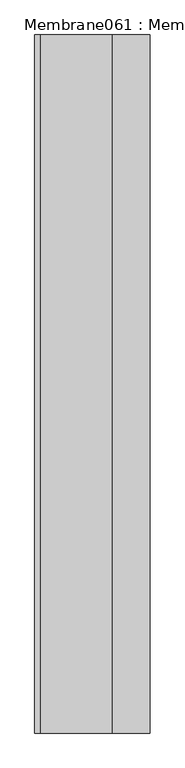
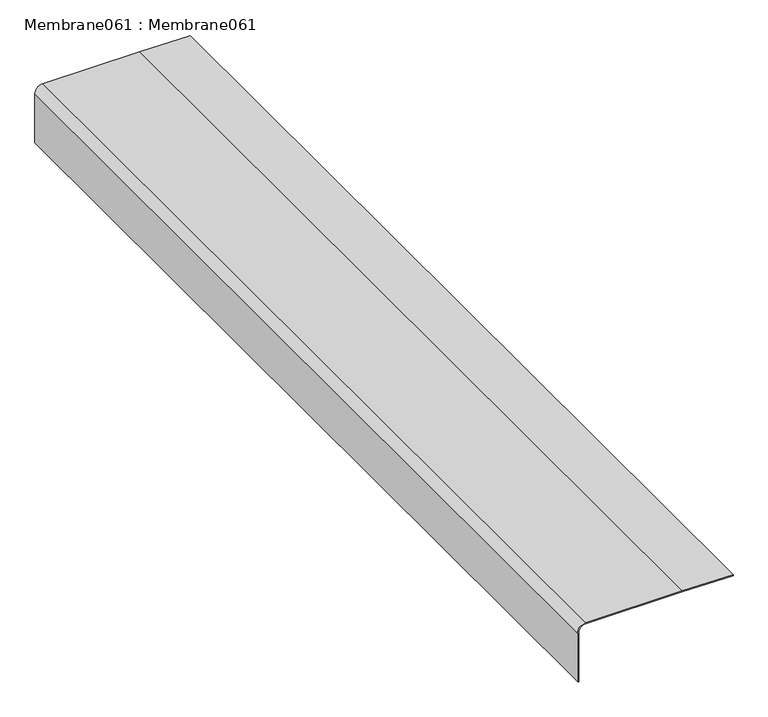
"""IFC4 building model written with IfcOpenShell, lengths in millimetres: proxy geometry, Membrane061 : Membrane061."""

import ifcopenshell
import ifcopenshell.guid

model = None  # the IFC model being written
_history = None  # IfcOwnerHistory: only IFC2X3 demands one
_inside = {}  # id of a spatial element -> (the spatial element, [elements in it])
_under = {}  # id of a project, library or spatial element -> (it, [spatial elements below it])
_declared = {}  # id of a project -> (the project, [libraries it declares])
_typed = {}  # id of a type object -> (the type object, [elements of that type])
_made_of = {}  # id of a material, layer set ... -> (it, [elements and type objects made of it])


def new_model(schema):
    """Start an empty IFC model of exactly this schema.

    Asked for "IFC4X3", IfcOpenShell would pick the latest addendum, in which some entities
    have other attributes; the version numbers below select the first issue.
    IFC2X3 requires an IfcOwnerHistory on every rooted entity: one is made here for all.
    """
    global model, _history
    if schema == "IFC4X3":
        model = ifcopenshell.file(schema_version=(4, 3, 0, 0))
    else:
        model = ifcopenshell.file(schema=schema)
    _inside.clear()
    _under.clear()
    _declared.clear()
    _typed.clear()
    _made_of.clear()
    _history = None
    if model.schema == "IFC2X3":
        org = make("IfcOrganization", Name="unknown")
        user = make(
            "IfcPersonAndOrganization",
            ThePerson=make("IfcPerson", FamilyName="unknown"),
            TheOrganization=org,
        )
        app = make(
            "IfcApplication",
            ApplicationDeveloper=org,
            Version="unknown",
            ApplicationFullName="unknown",
            ApplicationIdentifier="unknown",
        )
        _history = make(
            "IfcOwnerHistory",
            OwningUser=user,
            OwningApplication=app,
            ChangeAction="ADDED",
            CreationDate=0,
        )
    return model


def make(cls, **values):
    """One entity of the class cls with the attributes given. An attribute that is None is left unset."""
    return model.create_entity(
        cls, **{name: value for name, value in values.items() if value is not None}
    )


def rooted(cls, **values):
    """An entity with a GlobalId (a new one), such as an element, a storey or a relation."""
    return make(cls, GlobalId=ifcopenshell.guid.new(), OwnerHistory=_history, **values)


def si_unit(unit_type, name, prefix=None):
    """IfcSIUnit, for example si_unit("LENGTHUNIT", "METRE", prefix="MILLI")."""
    return make("IfcSIUnit", UnitType=unit_type, Prefix=prefix, Name=name)


def assignment(units):
    """IfcUnitAssignment: the units of a project."""
    return None if units is None else make("IfcUnitAssignment", Units=units)


def point(xyz):
    """IfcCartesianPoint."""
    return None if xyz is None else make("IfcCartesianPoint", Coordinates=xyz)


def direction(xyz):
    """IfcDirection."""
    return None if xyz is None else make("IfcDirection", DirectionRatios=xyz)


def frame(location, z_axis=None, x_axis=None):
    """IfcAxis2Placement3D, a coordinate frame: its origin and axes. An axis left out is left unset."""
    return make(
        "IfcAxis2Placement3D",
        Location=point(location),
        Axis=direction(z_axis),
        RefDirection=direction(x_axis),
    )


def frame_2d(location, x_axis=None):
    """IfcAxis2Placement2D, a coordinate frame in the plane: its origin and x axis."""
    return make(
        "IfcAxis2Placement2D", Location=point(location), RefDirection=direction(x_axis)
    )


def origin():
    """The frame at (0, 0, 0) with its axes left unset."""
    return frame((0.0, 0.0, 0.0))


def place(relative_to, where):
    """IfcLocalPlacement: puts the frame where relative to a parent placement (None: the world)."""
    return make(
        "IfcLocalPlacement", PlacementRelTo=relative_to, RelativePlacement=where
    )


def context(
    kind, dimensions, precision=None, world=None, true_north=None, identifier=None
):
    """IfcGeometricRepresentationContext, for example the 3D "Model" context."""
    return make(
        "IfcGeometricRepresentationContext",
        ContextIdentifier=identifier,
        ContextType=kind,
        CoordinateSpaceDimension=dimensions,
        Precision=precision,
        WorldCoordinateSystem=world,
        TrueNorth=true_north,
    )


def project(units=None, contexts=None):
    """IfcProject with its units and contexts."""
    return rooted(
        "IfcProject",
        Name="project",
        RepresentationContexts=contexts,
        UnitsInContext=assignment(units),
    )


def spatial(cls, under=None, at=None, **own):
    """A site, building, storey or space (cls), placed at a placement, below another one or the project."""
    s = rooted(cls, ObjectPlacement=at, **own)
    if under is not None:
        _under.setdefault(under.id(), (under, []))[1].append(s)
    return s


def polyline(points):
    """IfcPolyline through the points."""
    return make("IfcPolyline", Points=[point(p) for p in points])


def circle_curve(where, radius):
    """IfcCircle in the frame where."""
    return make("IfcCircle", Position=where, Radius=radius)


def trimmed(basis, trim1, trim2, sense, master):
    """IfcTrimmedCurve: the piece of a basis curve between two trims."""
    return make(
        "IfcTrimmedCurve",
        BasisCurve=basis,
        Trim1=trim1,
        Trim2=trim2,
        SenseAgreement=sense,
        MasterRepresentation=master,
    )


def segment(curve, same_sense, transition):
    """IfcCompositeCurveSegment."""
    return make(
        "IfcCompositeCurveSegment",
        Transition=transition,
        SameSense=same_sense,
        ParentCurve=curve,
    )


def composite_curve(segments, self_intersect=None):
    """IfcCompositeCurve: segments joined end to end."""
    return make("IfcCompositeCurve", Segments=segments, SelfIntersect=self_intersect)


def outline(outer, holes=None, kind="AREA"):
    """IfcArbitraryClosedProfileDef: a profile drawn as a closed curve; with holes, ...WithVoids."""
    if holes is None:
        return make("IfcArbitraryClosedProfileDef", ProfileType=kind, OuterCurve=outer)
    return make(
        "IfcArbitraryProfileDefWithVoids",
        ProfileType=kind,
        OuterCurve=outer,
        InnerCurves=holes,
    )


def extrude(swept, where, along, depth):
    """IfcExtrudedAreaSolid: the profile swept, set in the frame where, extruded along a direction by depth."""
    return make(
        "IfcExtrudedAreaSolid",
        SweptArea=swept,
        Position=where,
        ExtrudedDirection=direction(along),
        Depth=depth,
    )


def shape(context_of_items, identifier, shape_type, items):
    """IfcShapeRepresentation: the items that make up one representation, for example the "Body"."""
    return make(
        "IfcShapeRepresentation",
        ContextOfItems=context_of_items,
        RepresentationIdentifier=identifier,
        RepresentationType=shape_type,
        Items=items,
    )


def source(mapping_origin, context_of_items, identifier, shape_type, items):
    """IfcRepresentationMap: a shape defined once, which mapped items show again and again."""
    return make(
        "IfcRepresentationMap",
        MappingOrigin=mapping_origin,
        MappedRepresentation=shape(context_of_items, identifier, shape_type, items),
    )


def transform(
    local_origin,
    x_axis=None,
    y_axis=None,
    z_axis=None,
    scale=None,
    scale2=None,
    scale3=None,
    uniform=True,
):
    """IfcCartesianTransformationOperator3D, or its non-uniform kind. x_axis, y_axis, z_axis: its Axis1, 2, 3."""
    if uniform:
        return make(
            "IfcCartesianTransformationOperator3D",
            Axis1=direction(x_axis),
            Axis2=direction(y_axis),
            LocalOrigin=point(local_origin),
            Scale=scale,
            Axis3=direction(z_axis),
        )
    return make(
        "IfcCartesianTransformationOperator3DnonUniform",
        Axis1=direction(x_axis),
        Axis2=direction(y_axis),
        LocalOrigin=point(local_origin),
        Scale=scale,
        Axis3=direction(z_axis),
        Scale2=scale2,
        Scale3=scale3,
    )


def mapped(mapping_source, mapping_target):
    """IfcMappedItem: shows the shape of a source again, moved by a transform."""
    return make(
        "IfcMappedItem", MappingSource=mapping_source, MappingTarget=mapping_target
    )


def made_of(thing, what):
    """Note that an element or type object is made of a material, layer set ...; save() writes the relation."""
    if what is not None:
        _made_of.setdefault(what.id(), (what, []))[1].append(thing)
    return thing


def element(
    cls,
    number,
    at=None,
    inside=None,
    cuts=None,
    type_object=None,
    material=None,
    context=None,
    identifier="Body",
    shape_type=None,
    held_by="IfcProductDefinitionShape",
    body=None,
    shapes=None,
    **own,
):
    """One element of the class cls, such as IfcWall. Its Tag is "e" and its number.

    at: its placement. inside: the storey or other place that contains it. cuts: it is an
    opening in that element (IfcRelVoidsElement). A single representation is given by context,
    identifier, shape_type and body (its items); several are given by shapes. held_by: the class
    of the entity that holds the representations. save() writes the other relations.
    """
    e = rooted(cls, Tag="e%d" % number, ObjectPlacement=at, **own)
    if body is not None:
        shapes = [shape(context, identifier, shape_type, body)]
    if shapes is not None:
        e.Representation = make(held_by, Representations=shapes)
    if inside is not None:
        _inside.setdefault(inside.id(), (inside, []))[1].append(e)
    if cuts is not None:
        rooted(
            "IfcRelVoidsElement", RelatingBuildingElement=cuts, RelatedOpeningElement=e
        )
    if type_object is not None:
        _typed.setdefault(type_object.id(), (type_object, []))[1].append(e)
    return made_of(e, material)


def aggregate(whole, parts):
    """IfcRelAggregates: a whole, such as a stair, and the parts it consists of."""
    return rooted("IfcRelAggregates", RelatingObject=whole, RelatedObjects=parts)


def save(model, path):
    """Write the relations noted so far, then the file.

    IfcRelAggregates (storeys below a building ...), IfcRelContainedInSpatialStructure (elements
    in a storey), IfcRelDefinesByType, IfcRelAssociatesMaterial and IfcRelDeclares: one each for
    every whole, place, type object, material and project.
    """
    for whole, parts in _under.values():
        aggregate(whole, parts)
    for where, things in _inside.values():
        rooted(
            "IfcRelContainedInSpatialStructure",
            RelatedElements=things,
            RelatingStructure=where,
        )
    for kind, things in _typed.values():
        rooted("IfcRelDefinesByType", RelatedObjects=things, RelatingType=kind)
    for what, things in _made_of.values():
        rooted("IfcRelAssociatesMaterial", RelatedObjects=things, RelatingMaterial=what)
    for by, libraries in _declared.values():
        rooted("IfcRelDeclares", RelatingContext=by, RelatedDefinitions=libraries)
    model.write(path)


def membrane061_membrane061_8ba7ea15(model_context):
    return source(origin(), model_context, "Body", "SweptSolid", [
        extrude(outline(composite_curve([segment(trimmed(circle_curve(frame_2d((40234.8417335, -5013.5847849)), 15.0), [point((40234.8417335, -5028.5847849))], [point((40249.8417335, -5013.5847849))], True, "CARTESIAN"), True, "CONTINUOUS"), segment(polyline([(40249.8417335, -5013.5847849), (40249.8417335, -4807.9081377), (40248.2859925, -4699.8063764), (40250.2861996, -4699.8063764), (40251.8417335, -4807.893747), (40251.8417335, -5013.5847849)]), True, "CONTINUOUS"), segment(trimmed(circle_curve(frame_2d((40234.8417335, -5013.5847849)), 17.0), [point((40251.8417335, -5013.5847849))], [point((40234.8417335, -5030.5847849))], False, "CARTESIAN"), True, "CONTINUOUS"), segment(polyline([(40234.8417335, -5030.5847849), (40125.2457074, -5030.5847849), (40125.2457074, -5028.5847849), (40234.8417335, -5028.5847849)]), True, "CONTINUOUS")], self_intersect=False)), frame((0.0, -1052.8906574, 0.0), z_axis=(0.0, 1.0, 0.0), x_axis=(0.0, 0.0, 1.0)), (0.0, 0.0, 1.0), 2000.0),
    ])


if __name__ == "__main__":
    model = new_model("IFC4")
    model_context = context("Model", 3, world=origin())
    ifc_project = project(units=[si_unit("LENGTHUNIT", "METRE", prefix="MILLI")], contexts=[model_context])
    site = spatial("IfcSite", under=ifc_project)
    building = spatial("IfcBuilding", under=site)
    placement = place(None, origin())
    membrane061_membrane061_shape = membrane061_membrane061_8ba7ea15(model_context)
    element("IfcBuildingElementProxy", 1, Name="Membrane061 : Membrane061", ObjectType="Membrane061 : Membrane061", at=placement, inside=building, context=model_context, shape_type="MappedRepresentation", body=[
        mapped(membrane061_membrane061_shape, transform((0.0, 0.0, 0.0), x_axis=(1.0, 0.0, 0.0), y_axis=(0.0, 1.0, 0.0), z_axis=(0.0, 0.0, 1.0))),
    ])
    save(model, "model.ifc")

# Revit data of these elements
# Type "Membrane061 : Membrane061"
#   NameOverride = "Membrane061"
# Element 1 (IfcBuildingElementProxy, "Membrane061 : Membrane061")
#   Materials on its faces: "THREE PLY BUILT UP ROOF MEMBRANE"
# Materials
#   "THREE PLY BUILT UP ROOF MEMBRANE": class "Unassigned", colour RGB 63 63 63, transparency 0
